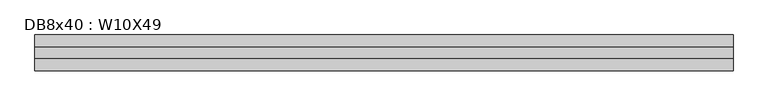
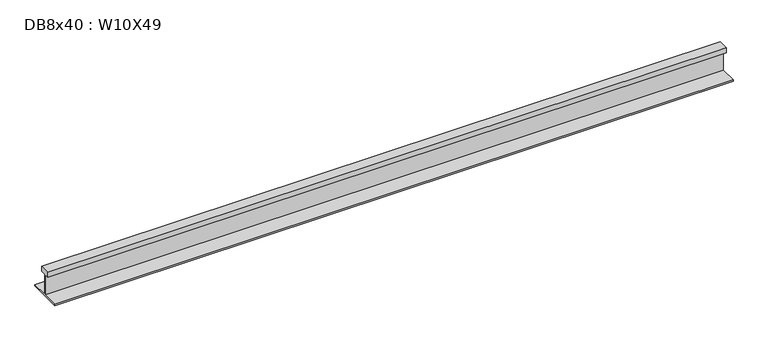
"""IFC4 building model written with IfcOpenShell, lengths in millimetres: beam geometry, DB8x40 : W10X49."""

import ifcopenshell
import ifcopenshell.guid

model = None  # the IFC model being written
_history = None  # IfcOwnerHistory: only IFC2X3 demands one
_inside = {}  # id of a spatial element -> (the spatial element, [elements in it])
_under = {}  # id of a project, library or spatial element -> (it, [spatial elements below it])
_declared = {}  # id of a project -> (the project, [libraries it declares])
_typed = {}  # id of a type object -> (the type object, [elements of that type])
_made_of = {}  # id of a material, layer set ... -> (it, [elements and type objects made of it])


def new_model(schema):
    """Start an empty IFC model of exactly this schema.

    Asked for "IFC4X3", IfcOpenShell would pick the latest addendum, in which some entities
    have other attributes; the version numbers below select the first issue.
    IFC2X3 requires an IfcOwnerHistory on every rooted entity: one is made here for all.
    """
    global model, _history
    if schema == "IFC4X3":
        model = ifcopenshell.file(schema_version=(4, 3, 0, 0))
    else:
        model = ifcopenshell.file(schema=schema)
    _inside.clear()
    _under.clear()
    _declared.clear()
    _typed.clear()
    _made_of.clear()
    _history = None
    if model.schema == "IFC2X3":
        org = make("IfcOrganization", Name="unknown")
        user = make(
            "IfcPersonAndOrganization",
            ThePerson=make("IfcPerson", FamilyName="unknown"),
            TheOrganization=org,
        )
        app = make(
            "IfcApplication",
            ApplicationDeveloper=org,
            Version="unknown",
            ApplicationFullName="unknown",
            ApplicationIdentifier="unknown",
        )
        _history = make(
            "IfcOwnerHistory",
            OwningUser=user,
            OwningApplication=app,
            ChangeAction="ADDED",
            CreationDate=0,
        )
    return model


def make(cls, **values):
    """One entity of the class cls with the attributes given. An attribute that is None is left unset."""
    return model.create_entity(
        cls, **{name: value for name, value in values.items() if value is not None}
    )


def rooted(cls, **values):
    """An entity with a GlobalId (a new one), such as an element, a storey or a relation."""
    return make(cls, GlobalId=ifcopenshell.guid.new(), OwnerHistory=_history, **values)


def si_unit(unit_type, name, prefix=None):
    """IfcSIUnit, for example si_unit("LENGTHUNIT", "METRE", prefix="MILLI")."""
    return make("IfcSIUnit", UnitType=unit_type, Prefix=prefix, Name=name)


def assignment(units):
    """IfcUnitAssignment: the units of a project."""
    return None if units is None else make("IfcUnitAssignment", Units=units)


def point(xyz):
    """IfcCartesianPoint."""
    return None if xyz is None else make("IfcCartesianPoint", Coordinates=xyz)


def direction(xyz):
    """IfcDirection."""
    return None if xyz is None else make("IfcDirection", DirectionRatios=xyz)


def frame(location, z_axis=None, x_axis=None):
    """IfcAxis2Placement3D, a coordinate frame: its origin and axes. An axis left out is left unset."""
    return make(
        "IfcAxis2Placement3D",
        Location=point(location),
        Axis=direction(z_axis),
        RefDirection=direction(x_axis),
    )


def origin():
    """The frame at (0, 0, 0) with its axes left unset."""
    return frame((0.0, 0.0, 0.0))


def place(relative_to, where):
    """IfcLocalPlacement: puts the frame where relative to a parent placement (None: the world)."""
    return make(
        "IfcLocalPlacement", PlacementRelTo=relative_to, RelativePlacement=where
    )


def context(
    kind, dimensions, precision=None, world=None, true_north=None, identifier=None
):
    """IfcGeometricRepresentationContext, for example the 3D "Model" context."""
    return make(
        "IfcGeometricRepresentationContext",
        ContextIdentifier=identifier,
        ContextType=kind,
        CoordinateSpaceDimension=dimensions,
        Precision=precision,
        WorldCoordinateSystem=world,
        TrueNorth=true_north,
    )


def project(units=None, contexts=None):
    """IfcProject with its units and contexts."""
    return rooted(
        "IfcProject",
        Name="project",
        RepresentationContexts=contexts,
        UnitsInContext=assignment(units),
    )


def spatial(cls, under=None, at=None, **own):
    """A site, building, storey or space (cls), placed at a placement, below another one or the project."""
    s = rooted(cls, ObjectPlacement=at, **own)
    if under is not None:
        _under.setdefault(under.id(), (under, []))[1].append(s)
    return s


def polyline(points):
    """IfcPolyline through the points."""
    return make("IfcPolyline", Points=[point(p) for p in points])


def outline(outer, holes=None, kind="AREA"):
    """IfcArbitraryClosedProfileDef: a profile drawn as a closed curve; with holes, ...WithVoids."""
    if holes is None:
        return make("IfcArbitraryClosedProfileDef", ProfileType=kind, OuterCurve=outer)
    return make(
        "IfcArbitraryProfileDefWithVoids",
        ProfileType=kind,
        OuterCurve=outer,
        InnerCurves=holes,
    )


def extrude(swept, where, along, depth):
    """IfcExtrudedAreaSolid: the profile swept, set in the frame where, extruded along a direction by depth."""
    return make(
        "IfcExtrudedAreaSolid",
        SweptArea=swept,
        Position=where,
        ExtrudedDirection=direction(along),
        Depth=depth,
    )


def shape(context_of_items, identifier, shape_type, items):
    """IfcShapeRepresentation: the items that make up one representation, for example the "Body"."""
    return make(
        "IfcShapeRepresentation",
        ContextOfItems=context_of_items,
        RepresentationIdentifier=identifier,
        RepresentationType=shape_type,
        Items=items,
    )


def source(mapping_origin, context_of_items, identifier, shape_type, items):
    """IfcRepresentationMap: a shape defined once, which mapped items show again and again."""
    return make(
        "IfcRepresentationMap",
        MappingOrigin=mapping_origin,
        MappedRepresentation=shape(context_of_items, identifier, shape_type, items),
    )


def transform(
    local_origin,
    x_axis=None,
    y_axis=None,
    z_axis=None,
    scale=None,
    scale2=None,
    scale3=None,
    uniform=True,
):
    """IfcCartesianTransformationOperator3D, or its non-uniform kind. x_axis, y_axis, z_axis: its Axis1, 2, 3."""
    if uniform:
        return make(
            "IfcCartesianTransformationOperator3D",
            Axis1=direction(x_axis),
            Axis2=direction(y_axis),
            LocalOrigin=point(local_origin),
            Scale=scale,
            Axis3=direction(z_axis),
        )
    return make(
        "IfcCartesianTransformationOperator3DnonUniform",
        Axis1=direction(x_axis),
        Axis2=direction(y_axis),
        LocalOrigin=point(local_origin),
        Scale=scale,
        Axis3=direction(z_axis),
        Scale2=scale2,
        Scale3=scale3,
    )


def mapped(mapping_source, mapping_target):
    """IfcMappedItem: shows the shape of a source again, moved by a transform."""
    return make(
        "IfcMappedItem", MappingSource=mapping_source, MappingTarget=mapping_target
    )


def made_of(thing, what):
    """Note that an element or type object is made of a material, layer set ...; save() writes the relation."""
    if what is not None:
        _made_of.setdefault(what.id(), (what, []))[1].append(thing)
    return thing


def element(
    cls,
    number,
    at=None,
    inside=None,
    cuts=None,
    type_object=None,
    material=None,
    context=None,
    identifier="Body",
    shape_type=None,
    held_by="IfcProductDefinitionShape",
    body=None,
    shapes=None,
    **own,
):
    """One element of the class cls, such as IfcWall. Its Tag is "e" and its number.

    at: its placement. inside: the storey or other place that contains it. cuts: it is an
    opening in that element (IfcRelVoidsElement). A single representation is given by context,
    identifier, shape_type and body (its items); several are given by shapes. held_by: the class
    of the entity that holds the representations. save() writes the other relations.
    """
    e = rooted(cls, Tag="e%d" % number, ObjectPlacement=at, **own)
    if body is not None:
        shapes = [shape(context, identifier, shape_type, body)]
    if shapes is not None:
        e.Representation = make(held_by, Representations=shapes)
    if inside is not None:
        _inside.setdefault(inside.id(), (inside, []))[1].append(e)
    if cuts is not None:
        rooted(
            "IfcRelVoidsElement", RelatingBuildingElement=cuts, RelatedOpeningElement=e
        )
    if type_object is not None:
        _typed.setdefault(type_object.id(), (type_object, []))[1].append(e)
    return made_of(e, material)


def aggregate(whole, parts):
    """IfcRelAggregates: a whole, such as a stair, and the parts it consists of."""
    return rooted("IfcRelAggregates", RelatingObject=whole, RelatedObjects=parts)


def save(model, path):
    """Write the relations noted so far, then the file.

    IfcRelAggregates (storeys below a building ...), IfcRelContainedInSpatialStructure (elements
    in a storey), IfcRelDefinesByType, IfcRelAssociatesMaterial and IfcRelDeclares: one each for
    every whole, place, type object, material and project.
    """
    for whole, parts in _under.values():
        aggregate(whole, parts)
    for where, things in _inside.values():
        rooted(
            "IfcRelContainedInSpatialStructure",
            RelatedElements=things,
            RelatingStructure=where,
        )
    for kind, things in _typed.values():
        rooted("IfcRelDefinesByType", RelatedObjects=things, RelatingType=kind)
    for what, things in _made_of.values():
        rooted("IfcRelAssociatesMaterial", RelatedObjects=things, RelatingMaterial=what)
    for by, libraries in _declared.values():
        rooted("IfcRelDeclares", RelatingContext=by, RelatedDefinitions=libraries)
    model.write(path)


def db8x40_w10x49_6679a255(model_context):
    return source(origin(), model_context, "Body", "SweptSolid", [
        extrude(outline(polyline([(38.1, 144.3355), (38.1, 106.2355), (2.921, 106.2355), (2.921, -49.53), (127.0, -49.53), (127.0, -59.182), (-127.0, -59.182), (-127.0, -49.53), (-2.921, -49.53), (-2.921, 106.2355), (-38.1, 106.2355), (-38.1, 144.3355), (38.1, 144.3355)])), frame((-2479.929, 0.0, 0.0), z_axis=(1.0, 0.0, 0.0), x_axis=(0.0, 1.0, 0.0)), (0.0, 0.0, 1.0), 4959.858),
    ])


if __name__ == "__main__":
    model = new_model("IFC4")
    model_context = context("Model", 3, world=origin())
    ifc_project = project(units=[si_unit("LENGTHUNIT", "METRE", prefix="MILLI")], contexts=[model_context])
    site = spatial("IfcSite", under=ifc_project)
    building = spatial("IfcBuilding", under=site)
    placement = place(None, origin())
    db8x40_w10x49_shape = db8x40_w10x49_6679a255(model_context)
    element("IfcBeam", 1, ObjectType="DB8x40 : W10X49", at=placement, inside=building, context=model_context, shape_type="MappedRepresentation", body=[
        mapped(db8x40_w10x49_shape, transform((0.0, 0.0, 0.0), x_axis=(1.0, 0.0, 0.0), y_axis=(0.0, 1.0, 0.0), z_axis=(0.0, 0.0, 1.0))),
    ])
    save(model, "model.ifc")

# Revit data of these elements
# Type "DB8x40 : W10X49"
#   Assembly Code = "B10"
#   W = 53
#   Length [instance default] = 5' - 0"
#   bf = 0' - 10"
#   d = 1' - 0.1"
#   k = 0' - 1 3/8"
#   k2 = 0' - 0.8"
#   tf = 0' - 0.575"
#   tw = 0' - 0.345"
#   A = 0.108333 SF
#   Structural Material [instance default] = Steel ASTM A992
# Element 1 (IfcBeam, "DB8x40 : W10X49")
#   Materials on its faces: "Steel ASTM A992"
# Materials
#   "Steel ASTM A992": class "Metal", colour RGB 199 199 199, transparency 0, Description = "Structural steel 50ksi", Cost = 0
